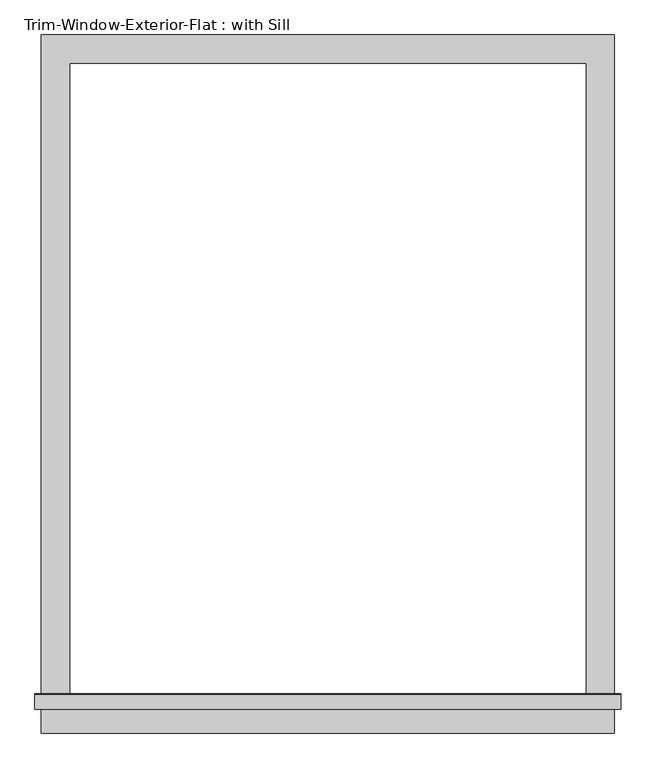
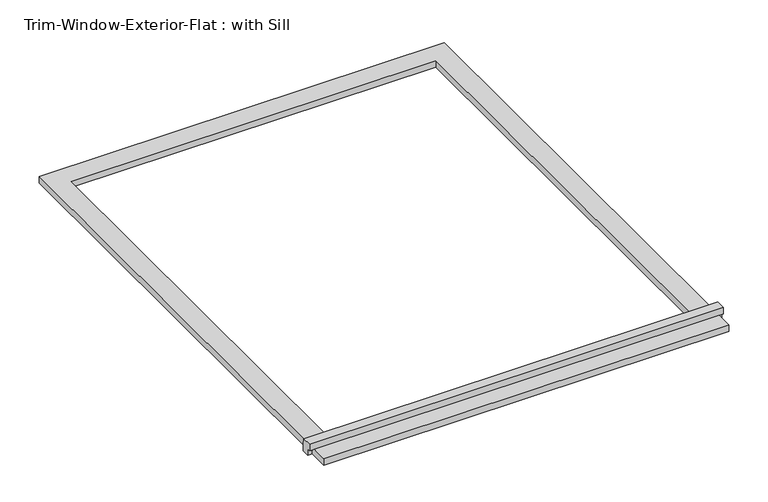
"""IFC4 building model written with IfcOpenShell, lengths in millimetres: proxy geometry, Trim-Window-Exterior-Flat : with Sill."""

from ifc_helpers import new_model, si_unit, frame, origin, origin_with_axes, place, context, project, spatial, polyline, outline, extrude, source, transform, mapped, element, save


def trim_window_exterior_flat_with_sill_1cb468f7(model_context):
    return source(origin(), model_context, "Body", "SweptSolid", [
        extrude(outline(polyline([(577.85, -1292.1823709), (577.85, -1349.3323709), (-577.85, -1349.3323709), (-577.85, -1292.1823709), (577.85, -1292.1823709)])), origin_with_axes(), (0.0, 0.0, 1.0), 19.05),
        extrude(outline(polyline([(-1301.75, 38.1), (-1272.4580645, 38.1), (-1270.0, 19.05), (-1270.0, 0.0), (-1292.1823709, 0.0), (-1292.1823709, 19.05), (-1301.75, 19.05), (-1301.75, 38.1)])), frame((-590.55, 0.0, 0.0), z_axis=(1.0, 0.0, 0.0), x_axis=(0.0, 1.0, 0.0)), (0.0, 0.0, 1.0), 1181.1),
        extrude(outline(polyline([(-577.85, 57.15), (577.85, 57.15), (577.85, -1270.0), (520.7, -1270.0), (520.7, 0.0), (-520.7, 0.0), (-520.7, -1270.0), (-577.85, -1270.0), (-577.85, 57.15)])), origin_with_axes(), (0.0, 0.0, 1.0), 19.05),
    ])


if __name__ == "__main__":
    model = new_model("IFC4")
    model_context = context("Model", 3, world=origin())
    ifc_project = project(units=[si_unit("LENGTHUNIT", "METRE", prefix="MILLI")], contexts=[model_context])
    site = spatial("IfcSite", under=ifc_project)
    building = spatial("IfcBuilding", under=site)
    placement = place(None, origin())
    trim_window_exterior_flat_with_sill_shape = trim_window_exterior_flat_with_sill_1cb468f7(model_context)
    element("IfcBuildingElementProxy", 1, Name="Trim-Window-Exterior-Flat : with Sill", ObjectType="Trim-Window-Exterior-Flat : with Sill", at=placement, inside=building, context=model_context, shape_type="MappedRepresentation", body=[
        mapped(trim_window_exterior_flat_with_sill_shape, transform((0.0, 0.0, 0.0), x_axis=(1.0, 0.0, 0.0), y_axis=(0.0, 1.0, 0.0), z_axis=(0.0, 0.0, 1.0))),
    ])
    save(model, "model.ifc")

# Revit data of these elements
# Type "Trim-Window-Exterior-Flat : with Sill"
#   Trim Width = 0' - 2 1/4"
#   Trim Thickness_Picture Frame = 0' - 1 1/4"
#   Trim Thickness_with Sill = 0' - 0 3/4"
#   Sill Thickness = 0' - 1 1/4"
#   Opening Width [instance default] = 2' - 0"
#   Opening Height [instance default] = 3' - 0"
#   Default Elevation = 4' - 0"
#   Sill = yes
#   Picture Frame = no
#   Trim Material [instance default] = none
# Element 1 (IfcBuildingElementProxy, "Trim-Window-Exterior-Flat : with Sill")
#   Opening Width = 3' - 5"
#   Opening Height = 4' - 2"
#   Trim Material = 1X WOOD COMPOSITE TRIM
#   Materials on its faces: "1X WOOD COMPOSITE TRIM"
# Materials
#   "1X WOOD COMPOSITE TRIM": class "Generic", colour RGB 88 61 61, transparency 0, Cost = 0
